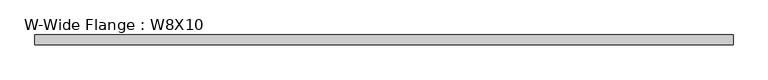
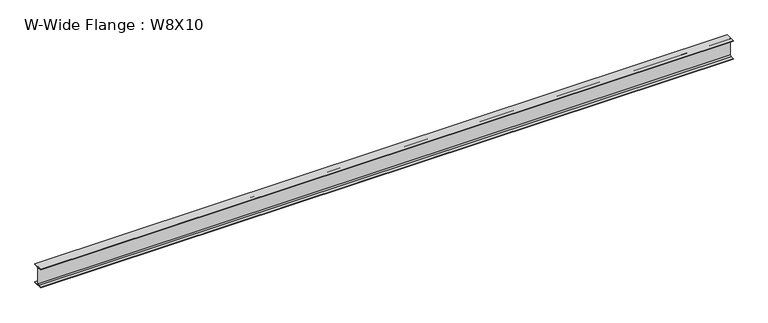
"""IFC4 building model written with IfcOpenShell, lengths in millimetres: beam geometry, W-Wide Flange : W8X10."""

from ifc_helpers import new_model, si_unit, point, frame, frame_2d, origin, place, context, project, spatial, polyline, circle_curve, trimmed, segment, composite_curve, outline, extrude, source, transform, mapped, element, save


def w_wide_flange_w8x10_eb5bcf21(model_context):
    return source(origin(), model_context, "Body", "SweptSolid", [
        extrude(outline(composite_curve([segment(polyline([(50.038, -94.996), (50.038, -100.203), (-50.038, -100.203), (-50.038, -94.996), (-14.4145, -94.996)]), True, "CONTINUOUS"), segment(trimmed(circle_curve(frame_2d((-14.4145, -82.7405)), 12.2555), [point((-14.4145, -94.996))], [point((-2.159, -82.7405))], True, "CARTESIAN"), True, "CONTINUOUS"), segment(polyline([(-2.159, -82.7405), (-2.159, 82.7405)]), True, "CONTINUOUS"), segment(trimmed(circle_curve(frame_2d((-14.4145, 82.7405)), 12.2555), [point((-2.159, 82.7405))], [point((-14.4145, 94.996))], True, "CARTESIAN"), True, "CONTINUOUS"), segment(polyline([(-14.4145, 94.996), (-50.038, 94.996), (-50.038, 100.203), (50.038, 100.203), (50.038, 94.996), (14.4145, 94.996)]), True, "CONTINUOUS"), segment(trimmed(circle_curve(frame_2d((14.4145, 82.7405)), 12.2555), [point((14.4145, 94.996))], [point((2.159, 82.7405))], True, "CARTESIAN"), True, "CONTINUOUS"), segment(polyline([(2.159, 82.7405), (2.159, -82.7405)]), True, "CONTINUOUS"), segment(trimmed(circle_curve(frame_2d((14.4145, -82.7405)), 12.2555), [point((2.159, -82.7405))], [point((14.4145, -94.996))], True, "CARTESIAN"), True, "CONTINUOUS"), segment(polyline([(14.4145, -94.996), (50.038, -94.996)]), True, "CONTINUOUS")], self_intersect=False)), frame((-3555.238, 0.0, 0.0), z_axis=(1.0, 0.0, 0.0), x_axis=(0.0, 1.0, 0.0)), (0.0, 0.0, 1.0), 7060.438),
    ])


if __name__ == "__main__":
    model = new_model("IFC4")
    model_context = context("Model", 3, world=origin())
    ifc_project = project(units=[si_unit("LENGTHUNIT", "METRE", prefix="MILLI")], contexts=[model_context])
    site = spatial("IfcSite", under=ifc_project)
    building = spatial("IfcBuilding", under=site)
    placement = place(None, origin())
    w_wide_flange_w8x10_shape = w_wide_flange_w8x10_eb5bcf21(model_context)
    element("IfcBeam", 1, ObjectType="W-Wide Flange : W8X10", at=placement, inside=building, context=model_context, shape_type="MappedRepresentation", body=[
        mapped(w_wide_flange_w8x10_shape, transform((0.0, 0.0, 0.0), x_axis=(1.0, 0.0, 0.0), y_axis=(0.0, 1.0, 0.0), z_axis=(0.0, 0.0, 1.0))),
    ])
    save(model, "model.ifc")

# Revit data of these elements
# Type "W-Wide Flange : W8X10"
#   Assembly Code = "B10"
#   W = 10
#   Length [instance default] = 5' - 0"
#   bf = 0' - 3.94"
#   d = 0' - 7.89"
#   k = 0' - 0 11/16"
#   k2 = 0' - 0.4825"
#   tf = 0' - 0.205"
#   tw = 0' - 0.17"
#   A = 0.0205556 SF
#   Structural Material [instance default] = Steel ASTM A992
# Element 1 (IfcBeam, "W-Wide Flange : W8X10")
#   Structural Material = none
# Materials
#   "Steel ASTM A992": class "Metal", colour RGB 189 187 185, transparency 0, Description = "Structural steel 50ksi", Cost = 0
